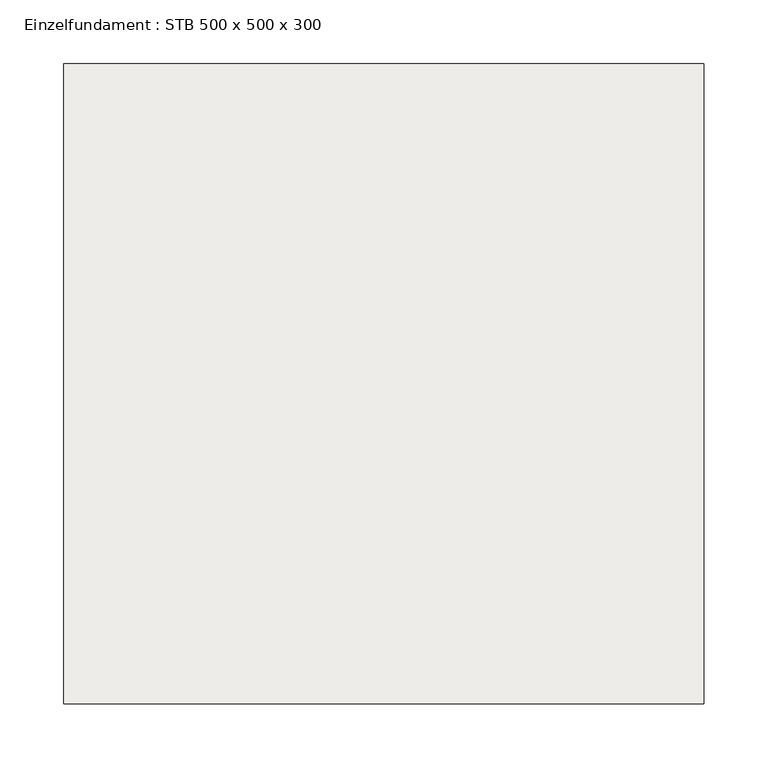
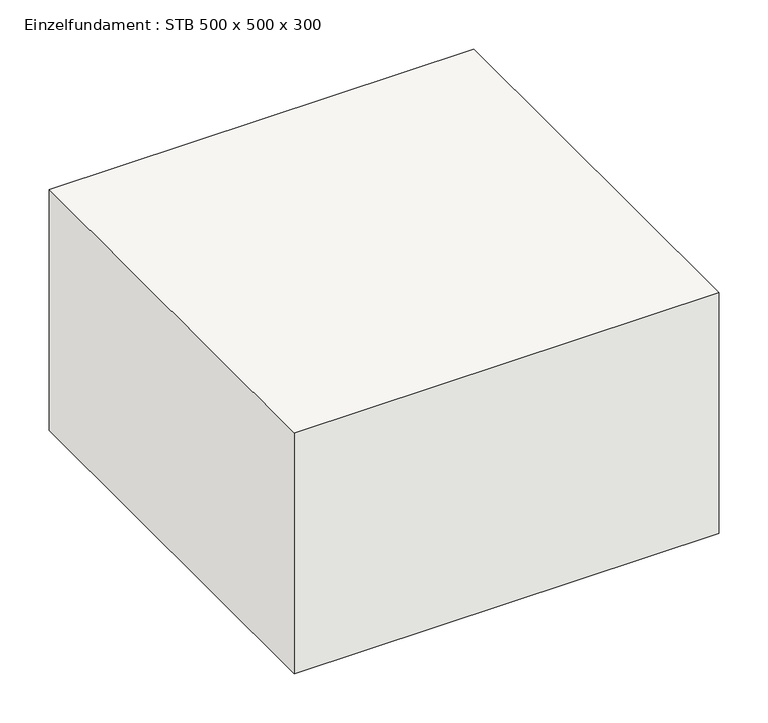
"""IFC4 building model written with IfcOpenShell, lengths in millimetres: slab geometry, Einzelfundament : STB 500 x 500 x 300."""

from ifc_helpers import new_model, si_unit, frame, origin, place, context, project, spatial, polyline, outline, extrude, source, transform, mapped, element, save


def einzelfundament_stb_500_x_500_x_300_3619195b(model_context):
    return source(origin(), model_context, "Body", "SweptSolid", [
        extrude(outline(polyline([(250.0, 250.0), (250.0, -250.0), (-250.0, -250.0), (-250.0, 250.0), (250.0, 250.0)])), frame((0.0, 0.0, -300.0), z_axis=(0.0, 0.0, 1.0), x_axis=(1.0, 0.0, 0.0)), (0.0, 0.0, 1.0), 300.0),
    ])


if __name__ == "__main__":
    model = new_model("IFC4")
    model_context = context("Model", 3, world=origin())
    ifc_project = project(units=[si_unit("LENGTHUNIT", "METRE", prefix="MILLI")], contexts=[model_context])
    site = spatial("IfcSite", under=ifc_project)
    building = spatial("IfcBuilding", under=site)
    placement = place(None, origin())
    einzelfundament_stb_500_x_500_x_300_shape = einzelfundament_stb_500_x_500_x_300_3619195b(model_context)
    element("IfcSlab", 1, ObjectType="Einzelfundament : STB 500 x 500 x 300", at=placement, inside=building, context=model_context, shape_type="MappedRepresentation", body=[
        mapped(einzelfundament_stb_500_x_500_x_300_shape, transform((0.0, 0.0, 0.0), x_axis=(1.0, 0.0, 0.0), y_axis=(0.0, 1.0, 0.0), z_axis=(0.0, 0.0, 1.0))),
    ])
    save(model, "model.ifc")

# Revit data of these elements
# Type "Einzelfundament : STB 500 x 500 x 300"
#   Type Comments = "L/B/H=50/50/30cm"
#   Punktbeschreibung [instance default] = ""
#   Description = "StB-Einzelfundament"
#   h = 0.300 m
#   ey [instance default] = 0.000 m
#   ex [instance default] = 0.000 m
#   by = 0.500 m
#   bx = 0.500 m
#   _ey [instance default] = 0.500 m
#   _ex [instance default] = 0.500 m
#   Length = 0.500 m
#   Höhe = 0.300 m
#   Foundation Thickness = 0.300 m
#   Width = 0.500 m
#   Structural Material = Ortbeton - unbewehrt
#   Assembly Code = ""
# Element 1 (IfcSlab, "Einzelfundament : STB 500 x 500 x 300")
#   Materials on its faces: "Ortbeton - unbewehrt"
# Materials
#   "Ortbeton - unbewehrt": class "Beton", colour RGB 189 189 189, transparency 0, Description = "Ortbeton - unbewehrt", Cost = 0
